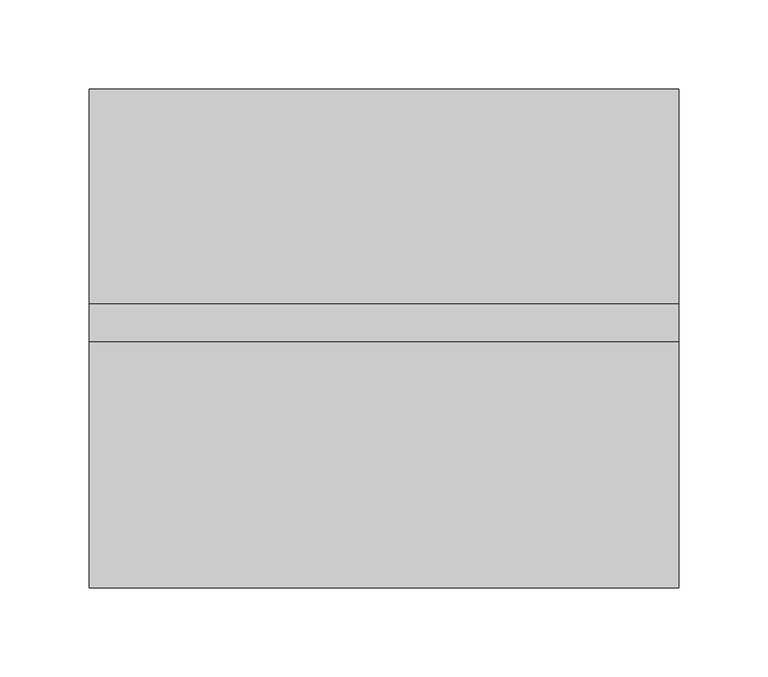
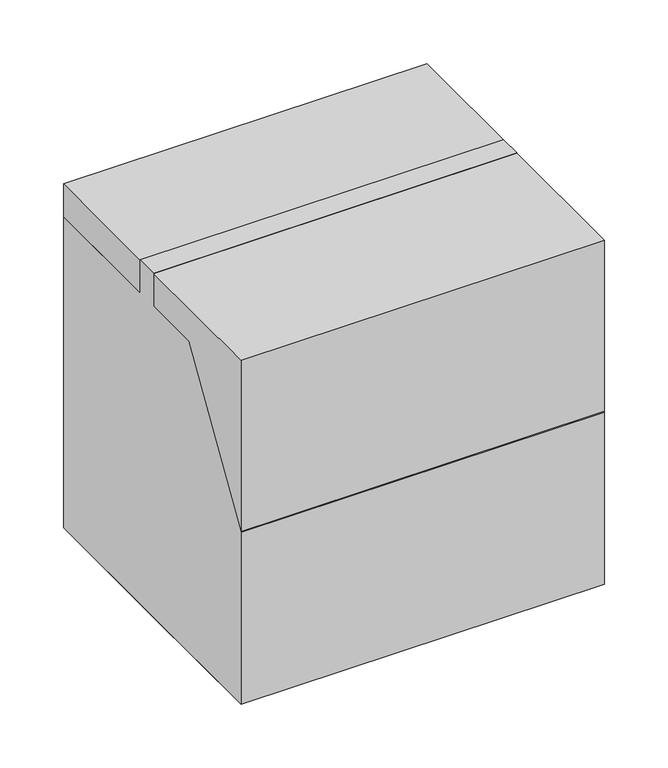
"""IFC4 building model written with IfcOpenShell, lengths in millimetres: proxy geometry, M4266 - Pump, Volumetric, Infusion, Multiple Line : M4266 - Pump, Volumetric, Infusion, Multiple Line."""

import ifcopenshell
import ifcopenshell.guid

model = None  # the IFC model being written
_history = None  # IfcOwnerHistory: only IFC2X3 demands one
_inside = {}  # id of a spatial element -> (the spatial element, [elements in it])
_under = {}  # id of a project, library or spatial element -> (it, [spatial elements below it])
_declared = {}  # id of a project -> (the project, [libraries it declares])
_typed = {}  # id of a type object -> (the type object, [elements of that type])
_made_of = {}  # id of a material, layer set ... -> (it, [elements and type objects made of it])


def new_model(schema):
    """Start an empty IFC model of exactly this schema.

    Asked for "IFC4X3", IfcOpenShell would pick the latest addendum, in which some entities
    have other attributes; the version numbers below select the first issue.
    IFC2X3 requires an IfcOwnerHistory on every rooted entity: one is made here for all.
    """
    global model, _history
    if schema == "IFC4X3":
        model = ifcopenshell.file(schema_version=(4, 3, 0, 0))
    else:
        model = ifcopenshell.file(schema=schema)
    _inside.clear()
    _under.clear()
    _declared.clear()
    _typed.clear()
    _made_of.clear()
    _history = None
    if model.schema == "IFC2X3":
        org = make("IfcOrganization", Name="unknown")
        user = make(
            "IfcPersonAndOrganization",
            ThePerson=make("IfcPerson", FamilyName="unknown"),
            TheOrganization=org,
        )
        app = make(
            "IfcApplication",
            ApplicationDeveloper=org,
            Version="unknown",
            ApplicationFullName="unknown",
            ApplicationIdentifier="unknown",
        )
        _history = make(
            "IfcOwnerHistory",
            OwningUser=user,
            OwningApplication=app,
            ChangeAction="ADDED",
            CreationDate=0,
        )
    return model


def make(cls, **values):
    """One entity of the class cls with the attributes given. An attribute that is None is left unset."""
    return model.create_entity(
        cls, **{name: value for name, value in values.items() if value is not None}
    )


def rooted(cls, **values):
    """An entity with a GlobalId (a new one), such as an element, a storey or a relation."""
    return make(cls, GlobalId=ifcopenshell.guid.new(), OwnerHistory=_history, **values)


def si_unit(unit_type, name, prefix=None):
    """IfcSIUnit, for example si_unit("LENGTHUNIT", "METRE", prefix="MILLI")."""
    return make("IfcSIUnit", UnitType=unit_type, Prefix=prefix, Name=name)


def assignment(units):
    """IfcUnitAssignment: the units of a project."""
    return None if units is None else make("IfcUnitAssignment", Units=units)


def point(xyz):
    """IfcCartesianPoint."""
    return None if xyz is None else make("IfcCartesianPoint", Coordinates=xyz)


def direction(xyz):
    """IfcDirection."""
    return None if xyz is None else make("IfcDirection", DirectionRatios=xyz)


def frame(location, z_axis=None, x_axis=None):
    """IfcAxis2Placement3D, a coordinate frame: its origin and axes. An axis left out is left unset."""
    return make(
        "IfcAxis2Placement3D",
        Location=point(location),
        Axis=direction(z_axis),
        RefDirection=direction(x_axis),
    )


def origin():
    """The frame at (0, 0, 0) with its axes left unset."""
    return frame((0.0, 0.0, 0.0))


def origin_with_axes():
    """The frame at (0, 0, 0) with the z axis (0, 0, 1) and the x axis (1, 0, 0) written out."""
    return frame((0.0, 0.0, 0.0), z_axis=(0.0, 0.0, 1.0), x_axis=(1.0, 0.0, 0.0))


def place(relative_to, where):
    """IfcLocalPlacement: puts the frame where relative to a parent placement (None: the world)."""
    return make(
        "IfcLocalPlacement", PlacementRelTo=relative_to, RelativePlacement=where
    )


def context(
    kind, dimensions, precision=None, world=None, true_north=None, identifier=None
):
    """IfcGeometricRepresentationContext, for example the 3D "Model" context."""
    return make(
        "IfcGeometricRepresentationContext",
        ContextIdentifier=identifier,
        ContextType=kind,
        CoordinateSpaceDimension=dimensions,
        Precision=precision,
        WorldCoordinateSystem=world,
        TrueNorth=true_north,
    )


def project(units=None, contexts=None):
    """IfcProject with its units and contexts."""
    return rooted(
        "IfcProject",
        Name="project",
        RepresentationContexts=contexts,
        UnitsInContext=assignment(units),
    )


def spatial(cls, under=None, at=None, **own):
    """A site, building, storey or space (cls), placed at a placement, below another one or the project."""
    s = rooted(cls, ObjectPlacement=at, **own)
    if under is not None:
        _under.setdefault(under.id(), (under, []))[1].append(s)
    return s


def polyline(points):
    """IfcPolyline through the points."""
    return make("IfcPolyline", Points=[point(p) for p in points])


def outline(outer, holes=None, kind="AREA"):
    """IfcArbitraryClosedProfileDef: a profile drawn as a closed curve; with holes, ...WithVoids."""
    if holes is None:
        return make("IfcArbitraryClosedProfileDef", ProfileType=kind, OuterCurve=outer)
    return make(
        "IfcArbitraryProfileDefWithVoids",
        ProfileType=kind,
        OuterCurve=outer,
        InnerCurves=holes,
    )


def extrude(swept, where, along, depth):
    """IfcExtrudedAreaSolid: the profile swept, set in the frame where, extruded along a direction by depth."""
    return make(
        "IfcExtrudedAreaSolid",
        SweptArea=swept,
        Position=where,
        ExtrudedDirection=direction(along),
        Depth=depth,
    )


def faces_of(points, faces, orient=None, outer=None):
    """IfcFace entities. A face is a list of loops; a loop is a list of indices into points, from 0.

    orient and outer hold one flag for each loop. By default every Orientation is true, the
    first loop of a face is its IfcFaceOuterBound and the others are IfcFaceBound.
    """
    made = []
    for i, loops in enumerate(faces):
        bounds = []
        for j, loop in enumerate(loops):
            is_outer = j == 0 if outer is None else outer[i][j]
            bounds.append(
                make(
                    "IfcFaceOuterBound" if is_outer else "IfcFaceBound",
                    Bound=make("IfcPolyLoop", Polygon=[points[k] for k in loop]),
                    Orientation=True if orient is None else orient[i][j],
                )
            )
        made.append(make("IfcFace", Bounds=bounds))
    return made


def faceted_brep(points, faces, orient=None, outer=None, voids=None):
    """IfcFacetedBrep: a solid bounded by flat faces; with voids (closed shells), ...WithVoids."""
    shared = [point(p) for p in points]
    hull = make("IfcClosedShell", CfsFaces=faces_of(shared, faces, orient, outer))
    if voids is None:
        return make("IfcFacetedBrep", Outer=hull)
    return make(
        "IfcFacetedBrepWithVoids",
        Outer=hull,
        Voids=[
            make(cls, CfsFaces=faces_of(shared, fs, o, b)) for cls, fs, o, b in voids
        ],
    )


def shape(context_of_items, identifier, shape_type, items):
    """IfcShapeRepresentation: the items that make up one representation, for example the "Body"."""
    return make(
        "IfcShapeRepresentation",
        ContextOfItems=context_of_items,
        RepresentationIdentifier=identifier,
        RepresentationType=shape_type,
        Items=items,
    )


def source(mapping_origin, context_of_items, identifier, shape_type, items):
    """IfcRepresentationMap: a shape defined once, which mapped items show again and again."""
    return make(
        "IfcRepresentationMap",
        MappingOrigin=mapping_origin,
        MappedRepresentation=shape(context_of_items, identifier, shape_type, items),
    )


def transform(
    local_origin,
    x_axis=None,
    y_axis=None,
    z_axis=None,
    scale=None,
    scale2=None,
    scale3=None,
    uniform=True,
):
    """IfcCartesianTransformationOperator3D, or its non-uniform kind. x_axis, y_axis, z_axis: its Axis1, 2, 3."""
    if uniform:
        return make(
            "IfcCartesianTransformationOperator3D",
            Axis1=direction(x_axis),
            Axis2=direction(y_axis),
            LocalOrigin=point(local_origin),
            Scale=scale,
            Axis3=direction(z_axis),
        )
    return make(
        "IfcCartesianTransformationOperator3DnonUniform",
        Axis1=direction(x_axis),
        Axis2=direction(y_axis),
        LocalOrigin=point(local_origin),
        Scale=scale,
        Axis3=direction(z_axis),
        Scale2=scale2,
        Scale3=scale3,
    )


def mapped(mapping_source, mapping_target):
    """IfcMappedItem: shows the shape of a source again, moved by a transform."""
    return make(
        "IfcMappedItem", MappingSource=mapping_source, MappingTarget=mapping_target
    )


def made_of(thing, what):
    """Note that an element or type object is made of a material, layer set ...; save() writes the relation."""
    if what is not None:
        _made_of.setdefault(what.id(), (what, []))[1].append(thing)
    return thing


def element(
    cls,
    number,
    at=None,
    inside=None,
    cuts=None,
    type_object=None,
    material=None,
    context=None,
    identifier="Body",
    shape_type=None,
    held_by="IfcProductDefinitionShape",
    body=None,
    shapes=None,
    **own,
):
    """One element of the class cls, such as IfcWall. Its Tag is "e" and its number.

    at: its placement. inside: the storey or other place that contains it. cuts: it is an
    opening in that element (IfcRelVoidsElement). A single representation is given by context,
    identifier, shape_type and body (its items); several are given by shapes. held_by: the class
    of the entity that holds the representations. save() writes the other relations.
    """
    e = rooted(cls, Tag="e%d" % number, ObjectPlacement=at, **own)
    if body is not None:
        shapes = [shape(context, identifier, shape_type, body)]
    if shapes is not None:
        e.Representation = make(held_by, Representations=shapes)
    if inside is not None:
        _inside.setdefault(inside.id(), (inside, []))[1].append(e)
    if cuts is not None:
        rooted(
            "IfcRelVoidsElement", RelatingBuildingElement=cuts, RelatedOpeningElement=e
        )
    if type_object is not None:
        _typed.setdefault(type_object.id(), (type_object, []))[1].append(e)
    return made_of(e, material)


def aggregate(whole, parts):
    """IfcRelAggregates: a whole, such as a stair, and the parts it consists of."""
    return rooted("IfcRelAggregates", RelatingObject=whole, RelatedObjects=parts)


def save(model, path):
    """Write the relations noted so far, then the file.

    IfcRelAggregates (storeys below a building ...), IfcRelContainedInSpatialStructure (elements
    in a storey), IfcRelDefinesByType, IfcRelAssociatesMaterial and IfcRelDeclares: one each for
    every whole, place, type object, material and project.
    """
    for whole, parts in _under.values():
        aggregate(whole, parts)
    for where, things in _inside.values():
        rooted(
            "IfcRelContainedInSpatialStructure",
            RelatedElements=things,
            RelatingStructure=where,
        )
    for kind, things in _typed.values():
        rooted("IfcRelDefinesByType", RelatedObjects=things, RelatingType=kind)
    for what, things in _made_of.values():
        rooted("IfcRelAssociatesMaterial", RelatedObjects=things, RelatingMaterial=what)
    for by, libraries in _declared.values():
        rooted("IfcRelDeclares", RelatingContext=by, RelatedDefinitions=libraries)
    model.write(path)


def specialty_equipment_4850f0ac(model_context):
    return source(origin(), model_context, "Body", "SolidModel", [
        faceted_brep([(165.1, 139.7, 0.0), (165.1, 139.7, 298.45), (165.1, 19.3829835, 298.45), (165.1, 19.3829835, 330.2), (165.1, -1.7923057, 330.2), (165.1, -1.7923057, 298.45), (165.1, -57.15, 298.45), (165.1, -139.7, 165.1), (165.1, -139.7, 0.0), (-165.1, 139.7, 0.0), (-165.1, -139.7, 0.0), (-165.1, -139.7, 165.1), (-165.1, -57.15, 298.45), (-165.1, -1.7923057, 298.45), (-165.1, -1.7923057, 330.2), (-165.1, 19.3829835, 330.2), (-165.1, 19.3829835, 298.45), (-165.1, 139.7, 298.45), (130.175, 19.3829835, 323.85), (-127.0, 19.3829835, 323.85), (-127.0, 19.3829835, 304.8), (130.175, 19.3829835, 304.8), (-127.0, -1.7923057, 323.85), (130.175, -1.7923057, 323.85), (130.175, -1.7923057, 304.8), (-127.0, -1.7923057, 304.8)], [[[0, 1, 2, 3, 4, 5, 6, 7, 8]], [[9, 10, 11, 12, 13, 14, 15, 16, 17]], [[1, 0, 9, 17]], [[2, 1, 17, 16]], [[3, 2, 16, 15], [18, 19, 20, 21]], [[4, 3, 15, 14]], [[5, 4, 14, 13], [22, 23, 24, 25]], [[6, 5, 13, 12]], [[7, 6, 12, 11]], [[8, 7, 11, 10]], [[0, 8, 10, 9]], [[22, 19, 18, 23]], [[19, 22, 25, 20]], [[20, 25, 24, 21]], [[23, 18, 21, 24]]]),
        extrude(outline(polyline([(-165.1, 139.7), (165.1, 139.7), (165.1, -139.7), (-165.1, -139.7), (-165.1, 0.0), (-165.1, 139.7)])), origin_with_axes(), (0.0, 0.0, 1.0), 330.2),
    ])


if __name__ == "__main__":
    model = new_model("IFC4")
    model_context = context("Model", 3, world=origin())
    ifc_project = project(units=[si_unit("LENGTHUNIT", "METRE", prefix="MILLI")], contexts=[model_context])
    site = spatial("IfcSite", under=ifc_project)
    building = spatial("IfcBuilding", under=site)
    placement = place(None, origin())
    specialty_equipment_shape = specialty_equipment_4850f0ac(model_context)
    element("IfcBuildingElementProxy", 1, Name="M4266 - Pump, Volumetric, Infusion, Multiple Line : M4266 - Pump, Volumetric, Infusion, Multiple Line", ObjectType="M4266 - Pump, Volumetric, Infusion, Multiple Line : M4266 - Pump, Volumetric, Infusion, Multiple Line", at=placement, inside=building, context=model_context, shape_type="MappedRepresentation", body=[
        mapped(specialty_equipment_shape, transform((0.0, 0.0, 0.0), x_axis=(1.0, 0.0, 0.0), y_axis=(0.0, 1.0, 0.0), z_axis=(0.0, 0.0, 1.0))),
    ])
    save(model, "model.ifc")

# Revit data of these elements
# Type "M4266 - Pump, Volumetric, Infusion, Multiple Line : M4266 - Pump, Volumetric, Infusion, Multiple Line"
#   Watts2 = "0"
#   Watts1 = "120"
#   Unit_Issue = "EA"
#   UTIL_6_Misc = "-"
#   UTIL_5_NonMedGas = "-"
#   UTIL_4_MiscGas = "-"
#   UTIL_3_MedGas = "-"
#   UTIL_2_Elec = "A"
#   UTIL_1_WaterDrain = "-"
#   Nomenclature = "Pump, Volumetric, Infusion, Multiple Line"
#   NSN = "6515"
#   Location [instance default] = ""
#   JSN = "M4266"
#   Fund_Source_VA = "-"
#   Fund_Source_Navy = "-"
#   Fund_Source_Army = "-"
#   Fund_Source_AF = "-"
#   ELEC_Volts2 = "0"
#   ELEC_Volts1 = "120"
#   ELEC_Phase2 = "0"
#   ELEC_Phase1 = "1"
#   ELEC_HertzSwitch = "0"
#   ELEC_HertzDependent = "1"
#   ELEC_Hertz = "60"
#   ELEC_Amps2 = "0"
#   ELEC_Amps1 = "1"
#   DetailDescription = "Volumetric infusion pump. Pump is self-regulating with automatic sensor and adjustable rate. Equipped with visual and audible alarms and up to 10 hour capacity battery. For the administration of a wide variety of therapeutic agents where precise control is required. Unit provides individual control to IV lines simultaneously."
#   CAT_VA = "C"
#   CAT_Navy = "C"
#   CAT_IHS = "-"
#   CAT_Army = "C"
#   CAT_AF = "C"
#   BTUperhour = "0"
#   Weight_IP = 18
#   DIM_Width_IP = 1' - 1"
#   DIM_Height_IP = 1' - 1"
#   DIM_Depth_IP = 0' - 11"
#   finish [instance default] = none
# Element 1 (IfcBuildingElementProxy, "M4266 - Pump, Volumetric, Infusion, Multiple Line : M4266 - Pump, Volumetric, Infusion, Multiple Line")
#   Location = "TRET3"
#   Materials on its faces: "EquipSpace"
# Materials
#   "EquipSpace": class "Unassigned", colour RGB 221 217 195, transparency 0.5
